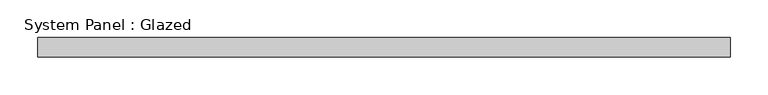
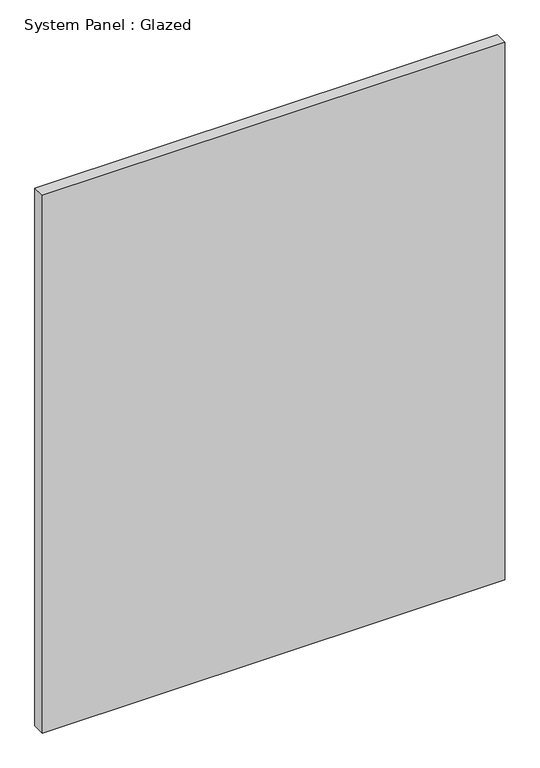
"""IFC4 building model written with IfcOpenShell, lengths in millimetres: plate geometry, System Panel : Glazed."""

import ifcopenshell
import ifcopenshell.guid

model = None  # the IFC model being written
_history = None  # IfcOwnerHistory: only IFC2X3 demands one
_inside = {}  # id of a spatial element -> (the spatial element, [elements in it])
_under = {}  # id of a project, library or spatial element -> (it, [spatial elements below it])
_declared = {}  # id of a project -> (the project, [libraries it declares])
_typed = {}  # id of a type object -> (the type object, [elements of that type])
_made_of = {}  # id of a material, layer set ... -> (it, [elements and type objects made of it])


def new_model(schema):
    """Start an empty IFC model of exactly this schema.

    Asked for "IFC4X3", IfcOpenShell would pick the latest addendum, in which some entities
    have other attributes; the version numbers below select the first issue.
    IFC2X3 requires an IfcOwnerHistory on every rooted entity: one is made here for all.
    """
    global model, _history
    if schema == "IFC4X3":
        model = ifcopenshell.file(schema_version=(4, 3, 0, 0))
    else:
        model = ifcopenshell.file(schema=schema)
    _inside.clear()
    _under.clear()
    _declared.clear()
    _typed.clear()
    _made_of.clear()
    _history = None
    if model.schema == "IFC2X3":
        org = make("IfcOrganization", Name="unknown")
        user = make(
            "IfcPersonAndOrganization",
            ThePerson=make("IfcPerson", FamilyName="unknown"),
            TheOrganization=org,
        )
        app = make(
            "IfcApplication",
            ApplicationDeveloper=org,
            Version="unknown",
            ApplicationFullName="unknown",
            ApplicationIdentifier="unknown",
        )
        _history = make(
            "IfcOwnerHistory",
            OwningUser=user,
            OwningApplication=app,
            ChangeAction="ADDED",
            CreationDate=0,
        )
    return model


def make(cls, **values):
    """One entity of the class cls with the attributes given. An attribute that is None is left unset."""
    return model.create_entity(
        cls, **{name: value for name, value in values.items() if value is not None}
    )


def rooted(cls, **values):
    """An entity with a GlobalId (a new one), such as an element, a storey or a relation."""
    return make(cls, GlobalId=ifcopenshell.guid.new(), OwnerHistory=_history, **values)


def si_unit(unit_type, name, prefix=None):
    """IfcSIUnit, for example si_unit("LENGTHUNIT", "METRE", prefix="MILLI")."""
    return make("IfcSIUnit", UnitType=unit_type, Prefix=prefix, Name=name)


def assignment(units):
    """IfcUnitAssignment: the units of a project."""
    return None if units is None else make("IfcUnitAssignment", Units=units)


def point(xyz):
    """IfcCartesianPoint."""
    return None if xyz is None else make("IfcCartesianPoint", Coordinates=xyz)


def direction(xyz):
    """IfcDirection."""
    return None if xyz is None else make("IfcDirection", DirectionRatios=xyz)


def frame(location, z_axis=None, x_axis=None):
    """IfcAxis2Placement3D, a coordinate frame: its origin and axes. An axis left out is left unset."""
    return make(
        "IfcAxis2Placement3D",
        Location=point(location),
        Axis=direction(z_axis),
        RefDirection=direction(x_axis),
    )


def origin():
    """The frame at (0, 0, 0) with its axes left unset."""
    return frame((0.0, 0.0, 0.0))


def origin_with_axes():
    """The frame at (0, 0, 0) with the z axis (0, 0, 1) and the x axis (1, 0, 0) written out."""
    return frame((0.0, 0.0, 0.0), z_axis=(0.0, 0.0, 1.0), x_axis=(1.0, 0.0, 0.0))


def place(relative_to, where):
    """IfcLocalPlacement: puts the frame where relative to a parent placement (None: the world)."""
    return make(
        "IfcLocalPlacement", PlacementRelTo=relative_to, RelativePlacement=where
    )


def context(
    kind, dimensions, precision=None, world=None, true_north=None, identifier=None
):
    """IfcGeometricRepresentationContext, for example the 3D "Model" context."""
    return make(
        "IfcGeometricRepresentationContext",
        ContextIdentifier=identifier,
        ContextType=kind,
        CoordinateSpaceDimension=dimensions,
        Precision=precision,
        WorldCoordinateSystem=world,
        TrueNorth=true_north,
    )


def project(units=None, contexts=None):
    """IfcProject with its units and contexts."""
    return rooted(
        "IfcProject",
        Name="project",
        RepresentationContexts=contexts,
        UnitsInContext=assignment(units),
    )


def spatial(cls, under=None, at=None, **own):
    """A site, building, storey or space (cls), placed at a placement, below another one or the project."""
    s = rooted(cls, ObjectPlacement=at, **own)
    if under is not None:
        _under.setdefault(under.id(), (under, []))[1].append(s)
    return s


def polyline(points):
    """IfcPolyline through the points."""
    return make("IfcPolyline", Points=[point(p) for p in points])


def outline(outer, holes=None, kind="AREA"):
    """IfcArbitraryClosedProfileDef: a profile drawn as a closed curve; with holes, ...WithVoids."""
    if holes is None:
        return make("IfcArbitraryClosedProfileDef", ProfileType=kind, OuterCurve=outer)
    return make(
        "IfcArbitraryProfileDefWithVoids",
        ProfileType=kind,
        OuterCurve=outer,
        InnerCurves=holes,
    )


def extrude(swept, where, along, depth):
    """IfcExtrudedAreaSolid: the profile swept, set in the frame where, extruded along a direction by depth."""
    return make(
        "IfcExtrudedAreaSolid",
        SweptArea=swept,
        Position=where,
        ExtrudedDirection=direction(along),
        Depth=depth,
    )


def shape(context_of_items, identifier, shape_type, items):
    """IfcShapeRepresentation: the items that make up one representation, for example the "Body"."""
    return make(
        "IfcShapeRepresentation",
        ContextOfItems=context_of_items,
        RepresentationIdentifier=identifier,
        RepresentationType=shape_type,
        Items=items,
    )


def source(mapping_origin, context_of_items, identifier, shape_type, items):
    """IfcRepresentationMap: a shape defined once, which mapped items show again and again."""
    return make(
        "IfcRepresentationMap",
        MappingOrigin=mapping_origin,
        MappedRepresentation=shape(context_of_items, identifier, shape_type, items),
    )


def transform(
    local_origin,
    x_axis=None,
    y_axis=None,
    z_axis=None,
    scale=None,
    scale2=None,
    scale3=None,
    uniform=True,
):
    """IfcCartesianTransformationOperator3D, or its non-uniform kind. x_axis, y_axis, z_axis: its Axis1, 2, 3."""
    if uniform:
        return make(
            "IfcCartesianTransformationOperator3D",
            Axis1=direction(x_axis),
            Axis2=direction(y_axis),
            LocalOrigin=point(local_origin),
            Scale=scale,
            Axis3=direction(z_axis),
        )
    return make(
        "IfcCartesianTransformationOperator3DnonUniform",
        Axis1=direction(x_axis),
        Axis2=direction(y_axis),
        LocalOrigin=point(local_origin),
        Scale=scale,
        Axis3=direction(z_axis),
        Scale2=scale2,
        Scale3=scale3,
    )


def mapped(mapping_source, mapping_target):
    """IfcMappedItem: shows the shape of a source again, moved by a transform."""
    return make(
        "IfcMappedItem", MappingSource=mapping_source, MappingTarget=mapping_target
    )


def made_of(thing, what):
    """Note that an element or type object is made of a material, layer set ...; save() writes the relation."""
    if what is not None:
        _made_of.setdefault(what.id(), (what, []))[1].append(thing)
    return thing


def element(
    cls,
    number,
    at=None,
    inside=None,
    cuts=None,
    type_object=None,
    material=None,
    context=None,
    identifier="Body",
    shape_type=None,
    held_by="IfcProductDefinitionShape",
    body=None,
    shapes=None,
    **own,
):
    """One element of the class cls, such as IfcWall. Its Tag is "e" and its number.

    at: its placement. inside: the storey or other place that contains it. cuts: it is an
    opening in that element (IfcRelVoidsElement). A single representation is given by context,
    identifier, shape_type and body (its items); several are given by shapes. held_by: the class
    of the entity that holds the representations. save() writes the other relations.
    """
    e = rooted(cls, Tag="e%d" % number, ObjectPlacement=at, **own)
    if body is not None:
        shapes = [shape(context, identifier, shape_type, body)]
    if shapes is not None:
        e.Representation = make(held_by, Representations=shapes)
    if inside is not None:
        _inside.setdefault(inside.id(), (inside, []))[1].append(e)
    if cuts is not None:
        rooted(
            "IfcRelVoidsElement", RelatingBuildingElement=cuts, RelatedOpeningElement=e
        )
    if type_object is not None:
        _typed.setdefault(type_object.id(), (type_object, []))[1].append(e)
    return made_of(e, material)


def aggregate(whole, parts):
    """IfcRelAggregates: a whole, such as a stair, and the parts it consists of."""
    return rooted("IfcRelAggregates", RelatingObject=whole, RelatedObjects=parts)


def save(model, path):
    """Write the relations noted so far, then the file.

    IfcRelAggregates (storeys below a building ...), IfcRelContainedInSpatialStructure (elements
    in a storey), IfcRelDefinesByType, IfcRelAssociatesMaterial and IfcRelDeclares: one each for
    every whole, place, type object, material and project.
    """
    for whole, parts in _under.values():
        aggregate(whole, parts)
    for where, things in _inside.values():
        rooted(
            "IfcRelContainedInSpatialStructure",
            RelatedElements=things,
            RelatingStructure=where,
        )
    for kind, things in _typed.values():
        rooted("IfcRelDefinesByType", RelatedObjects=things, RelatingType=kind)
    for what, things in _made_of.values():
        rooted("IfcRelAssociatesMaterial", RelatedObjects=things, RelatingMaterial=what)
    for by, libraries in _declared.values():
        rooted("IfcRelDeclares", RelatingContext=by, RelatedDefinitions=libraries)
    model.write(path)


def system_panel_glazed_2e5f6ce9(model_context):
    return source(origin(), model_context, "Body", "SweptSolid", [
        extrude(outline(polyline([(457.2, -44.45), (-457.2, -44.45), (-457.2, -19.05), (457.2, -19.05), (457.2, -44.45)])), origin_with_axes(), (0.0, 0.0, 1.0), 1123.95),
    ])


if __name__ == "__main__":
    model = new_model("IFC4")
    model_context = context("Model", 3, world=origin())
    ifc_project = project(units=[si_unit("LENGTHUNIT", "METRE", prefix="MILLI")], contexts=[model_context])
    site = spatial("IfcSite", under=ifc_project)
    building = spatial("IfcBuilding", under=site)
    placement = place(None, origin())
    system_panel_glazed_shape = system_panel_glazed_2e5f6ce9(model_context)
    element("IfcPlate", 1, ObjectType="System Panel : Glazed", at=placement, inside=building, context=model_context, shape_type="MappedRepresentation", body=[
        mapped(system_panel_glazed_shape, transform((0.0, 0.0, 0.0), x_axis=(1.0, 0.0, 0.0), y_axis=(0.0, 1.0, 0.0), z_axis=(0.0, 0.0, 1.0))),
    ])
    save(model, "model.ifc")

# Revit data of these elements
# Element 1 (IfcPlate, "System Panel : Glazed")
#   Materials on its faces: "Glass"
# Materials
#   "Glass": class "Glass", colour RGB 0 128 192, transparency 0.75
